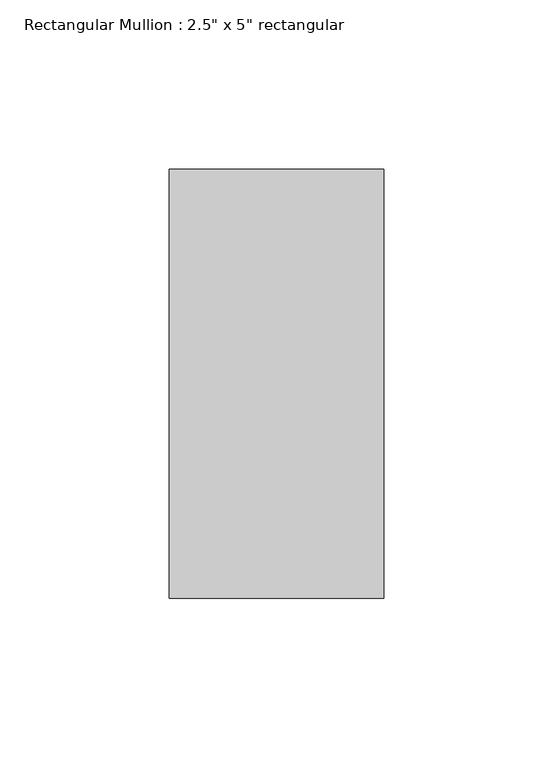
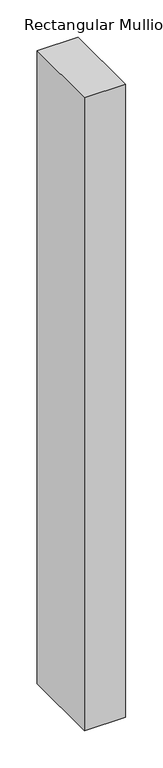
"""IFC4 building model written with IfcOpenShell, lengths in millimetres: member geometry."""

from ifc_helpers import new_model, si_unit, frame, origin, place, context, project, spatial, polyline, outline, extrude, source, transform, mapped, element, save


def member_309cb93c(model_context):
    return source(origin(), model_context, "Body", "SweptSolid", [
        extrude(outline(polyline([(31.75, 63.5), (31.75, -63.5), (-31.75, -63.5), (-31.75, 63.5), (31.75, 63.5)])), frame((0.0, 0.0, -1035.05), z_axis=(0.0, 0.0, 1.0), x_axis=(1.0, 0.0, 0.0)), (0.0, 0.0, 1.0), 1035.05),
    ])


if __name__ == "__main__":
    model = new_model("IFC4")
    model_context = context("Model", 3, world=origin())
    ifc_project = project(units=[si_unit("LENGTHUNIT", "METRE", prefix="MILLI")], contexts=[model_context])
    site = spatial("IfcSite", under=ifc_project)
    building = spatial("IfcBuilding", under=site)
    placement = place(None, origin())
    member_shape = member_309cb93c(model_context)
    element("IfcMember", 1, ObjectType="Rectangular Mullion : 2.5\" x 5\" rectangular", at=placement, inside=building, context=model_context, shape_type="MappedRepresentation", body=[
        mapped(member_shape, transform((0.0, 0.0, 0.0), x_axis=(1.0, 0.0, 0.0), y_axis=(0.0, 1.0, 0.0), z_axis=(0.0, 0.0, 1.0))),
    ])
    save(model, "model.ifc")

# Revit data of these elements
# Type "Rectangular Mullion : 2.5\" x 5\" rectangular"
#   built-in parameter 1007304 = 0.416667 (stored number, unit not read)
#   built-in parameter 1007301 = 0.104167 (stored number, unit not read)
#   built-in parameter 1007300 = 0.104167 (stored number, unit not read)
# Element 1 (IfcMember, "Rectangular Mullion : 2.5\" x 5\" rectangular")
#   Materials on its faces: "Metal - Aluminum"
# Materials
#   "Metal - Aluminum": class "Metal", colour RGB 140 140 140, transparency 0
